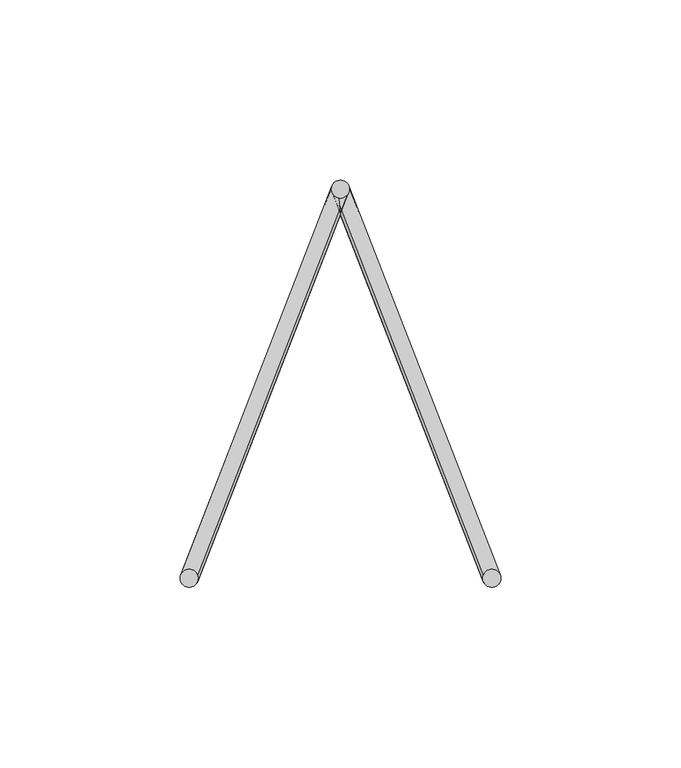
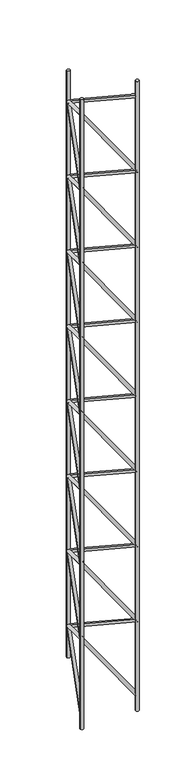
"""IFC4 building model written with IfcOpenShell, lengths in millimetres: proxy geometry, Pre-fab. (Vigota 4 - Pano 6)."""

import ifcopenshell
import ifcopenshell.guid

model = None  # the IFC model being written
_history = None  # IfcOwnerHistory: only IFC2X3 demands one
_inside = {}  # id of a spatial element -> (the spatial element, [elements in it])
_under = {}  # id of a project, library or spatial element -> (it, [spatial elements below it])
_declared = {}  # id of a project -> (the project, [libraries it declares])
_typed = {}  # id of a type object -> (the type object, [elements of that type])
_made_of = {}  # id of a material, layer set ... -> (it, [elements and type objects made of it])


def new_model(schema):
    """Start an empty IFC model of exactly this schema.

    Asked for "IFC4X3", IfcOpenShell would pick the latest addendum, in which some entities
    have other attributes; the version numbers below select the first issue.
    IFC2X3 requires an IfcOwnerHistory on every rooted entity: one is made here for all.
    """
    global model, _history
    if schema == "IFC4X3":
        model = ifcopenshell.file(schema_version=(4, 3, 0, 0))
    else:
        model = ifcopenshell.file(schema=schema)
    _inside.clear()
    _under.clear()
    _declared.clear()
    _typed.clear()
    _made_of.clear()
    _history = None
    if model.schema == "IFC2X3":
        org = make("IfcOrganization", Name="unknown")
        user = make(
            "IfcPersonAndOrganization",
            ThePerson=make("IfcPerson", FamilyName="unknown"),
            TheOrganization=org,
        )
        app = make(
            "IfcApplication",
            ApplicationDeveloper=org,
            Version="unknown",
            ApplicationFullName="unknown",
            ApplicationIdentifier="unknown",
        )
        _history = make(
            "IfcOwnerHistory",
            OwningUser=user,
            OwningApplication=app,
            ChangeAction="ADDED",
            CreationDate=0,
        )
    return model


def make(cls, **values):
    """One entity of the class cls with the attributes given. An attribute that is None is left unset."""
    return model.create_entity(
        cls, **{name: value for name, value in values.items() if value is not None}
    )


def rooted(cls, **values):
    """An entity with a GlobalId (a new one), such as an element, a storey or a relation."""
    return make(cls, GlobalId=ifcopenshell.guid.new(), OwnerHistory=_history, **values)


def si_unit(unit_type, name, prefix=None):
    """IfcSIUnit, for example si_unit("LENGTHUNIT", "METRE", prefix="MILLI")."""
    return make("IfcSIUnit", UnitType=unit_type, Prefix=prefix, Name=name)


def assignment(units):
    """IfcUnitAssignment: the units of a project."""
    return None if units is None else make("IfcUnitAssignment", Units=units)


def point(xyz):
    """IfcCartesianPoint."""
    return None if xyz is None else make("IfcCartesianPoint", Coordinates=xyz)


def direction(xyz):
    """IfcDirection."""
    return None if xyz is None else make("IfcDirection", DirectionRatios=xyz)


def frame(location, z_axis=None, x_axis=None):
    """IfcAxis2Placement3D, a coordinate frame: its origin and axes. An axis left out is left unset."""
    return make(
        "IfcAxis2Placement3D",
        Location=point(location),
        Axis=direction(z_axis),
        RefDirection=direction(x_axis),
    )


def frame_2d(location, x_axis=None):
    """IfcAxis2Placement2D, a coordinate frame in the plane: its origin and x axis."""
    return make(
        "IfcAxis2Placement2D", Location=point(location), RefDirection=direction(x_axis)
    )


def origin():
    """The frame at (0, 0, 0) with its axes left unset."""
    return frame((0.0, 0.0, 0.0))


def origin_with_axes():
    """The frame at (0, 0, 0) with the z axis (0, 0, 1) and the x axis (1, 0, 0) written out."""
    return frame((0.0, 0.0, 0.0), z_axis=(0.0, 0.0, 1.0), x_axis=(1.0, 0.0, 0.0))


def origin_2d():
    """The frame at (0, 0) in the plane with its x axis left unset."""
    return frame_2d((0.0, 0.0))


def place(relative_to, where):
    """IfcLocalPlacement: puts the frame where relative to a parent placement (None: the world)."""
    return make(
        "IfcLocalPlacement", PlacementRelTo=relative_to, RelativePlacement=where
    )


def context(
    kind, dimensions, precision=None, world=None, true_north=None, identifier=None
):
    """IfcGeometricRepresentationContext, for example the 3D "Model" context."""
    return make(
        "IfcGeometricRepresentationContext",
        ContextIdentifier=identifier,
        ContextType=kind,
        CoordinateSpaceDimension=dimensions,
        Precision=precision,
        WorldCoordinateSystem=world,
        TrueNorth=true_north,
    )


def project(units=None, contexts=None):
    """IfcProject with its units and contexts."""
    return rooted(
        "IfcProject",
        Name="project",
        RepresentationContexts=contexts,
        UnitsInContext=assignment(units),
    )


def spatial(cls, under=None, at=None, **own):
    """A site, building, storey or space (cls), placed at a placement, below another one or the project."""
    s = rooted(cls, ObjectPlacement=at, **own)
    if under is not None:
        _under.setdefault(under.id(), (under, []))[1].append(s)
    return s


def circle_curve(where, radius):
    """IfcCircle in the frame where."""
    return make("IfcCircle", Position=where, Radius=radius)


def trimmed(basis, trim1, trim2, sense, master):
    """IfcTrimmedCurve: the piece of a basis curve between two trims."""
    return make(
        "IfcTrimmedCurve",
        BasisCurve=basis,
        Trim1=trim1,
        Trim2=trim2,
        SenseAgreement=sense,
        MasterRepresentation=master,
    )


def segment(curve, same_sense, transition):
    """IfcCompositeCurveSegment."""
    return make(
        "IfcCompositeCurveSegment",
        Transition=transition,
        SameSense=same_sense,
        ParentCurve=curve,
    )


def composite_curve(segments, self_intersect=None):
    """IfcCompositeCurve: segments joined end to end."""
    return make("IfcCompositeCurve", Segments=segments, SelfIntersect=self_intersect)


def outline(outer, holes=None, kind="AREA"):
    """IfcArbitraryClosedProfileDef: a profile drawn as a closed curve; with holes, ...WithVoids."""
    if holes is None:
        return make("IfcArbitraryClosedProfileDef", ProfileType=kind, OuterCurve=outer)
    return make(
        "IfcArbitraryProfileDefWithVoids",
        ProfileType=kind,
        OuterCurve=outer,
        InnerCurves=holes,
    )


def extrude(swept, where, along, depth):
    """IfcExtrudedAreaSolid: the profile swept, set in the frame where, extruded along a direction by depth."""
    return make(
        "IfcExtrudedAreaSolid",
        SweptArea=swept,
        Position=where,
        ExtrudedDirection=direction(along),
        Depth=depth,
    )


def shape(context_of_items, identifier, shape_type, items):
    """IfcShapeRepresentation: the items that make up one representation, for example the "Body"."""
    return make(
        "IfcShapeRepresentation",
        ContextOfItems=context_of_items,
        RepresentationIdentifier=identifier,
        RepresentationType=shape_type,
        Items=items,
    )


def source(mapping_origin, context_of_items, identifier, shape_type, items):
    """IfcRepresentationMap: a shape defined once, which mapped items show again and again."""
    return make(
        "IfcRepresentationMap",
        MappingOrigin=mapping_origin,
        MappedRepresentation=shape(context_of_items, identifier, shape_type, items),
    )


def transform(
    local_origin,
    x_axis=None,
    y_axis=None,
    z_axis=None,
    scale=None,
    scale2=None,
    scale3=None,
    uniform=True,
):
    """IfcCartesianTransformationOperator3D, or its non-uniform kind. x_axis, y_axis, z_axis: its Axis1, 2, 3."""
    if uniform:
        return make(
            "IfcCartesianTransformationOperator3D",
            Axis1=direction(x_axis),
            Axis2=direction(y_axis),
            LocalOrigin=point(local_origin),
            Scale=scale,
            Axis3=direction(z_axis),
        )
    return make(
        "IfcCartesianTransformationOperator3DnonUniform",
        Axis1=direction(x_axis),
        Axis2=direction(y_axis),
        LocalOrigin=point(local_origin),
        Scale=scale,
        Axis3=direction(z_axis),
        Scale2=scale2,
        Scale3=scale3,
    )


def mapped(mapping_source, mapping_target):
    """IfcMappedItem: shows the shape of a source again, moved by a transform."""
    return make(
        "IfcMappedItem", MappingSource=mapping_source, MappingTarget=mapping_target
    )


def made_of(thing, what):
    """Note that an element or type object is made of a material, layer set ...; save() writes the relation."""
    if what is not None:
        _made_of.setdefault(what.id(), (what, []))[1].append(thing)
    return thing


def element(
    cls,
    number,
    at=None,
    inside=None,
    cuts=None,
    type_object=None,
    material=None,
    context=None,
    identifier="Body",
    shape_type=None,
    held_by="IfcProductDefinitionShape",
    body=None,
    shapes=None,
    **own,
):
    """One element of the class cls, such as IfcWall. Its Tag is "e" and its number.

    at: its placement. inside: the storey or other place that contains it. cuts: it is an
    opening in that element (IfcRelVoidsElement). A single representation is given by context,
    identifier, shape_type and body (its items); several are given by shapes. held_by: the class
    of the entity that holds the representations. save() writes the other relations.
    """
    e = rooted(cls, Tag="e%d" % number, ObjectPlacement=at, **own)
    if body is not None:
        shapes = [shape(context, identifier, shape_type, body)]
    if shapes is not None:
        e.Representation = make(held_by, Representations=shapes)
    if inside is not None:
        _inside.setdefault(inside.id(), (inside, []))[1].append(e)
    if cuts is not None:
        rooted(
            "IfcRelVoidsElement", RelatingBuildingElement=cuts, RelatedOpeningElement=e
        )
    if type_object is not None:
        _typed.setdefault(type_object.id(), (type_object, []))[1].append(e)
    return made_of(e, material)


def aggregate(whole, parts):
    """IfcRelAggregates: a whole, such as a stair, and the parts it consists of."""
    return rooted("IfcRelAggregates", RelatingObject=whole, RelatedObjects=parts)


def save(model, path):
    """Write the relations noted so far, then the file.

    IfcRelAggregates (storeys below a building ...), IfcRelContainedInSpatialStructure (elements
    in a storey), IfcRelDefinesByType, IfcRelAssociatesMaterial and IfcRelDeclares: one each for
    every whole, place, type object, material and project.
    """
    for whole, parts in _under.values():
        aggregate(whole, parts)
    for where, things in _inside.values():
        rooted(
            "IfcRelContainedInSpatialStructure",
            RelatedElements=things,
            RelatingStructure=where,
        )
    for kind, things in _typed.values():
        rooted("IfcRelDefinesByType", RelatedObjects=things, RelatingType=kind)
    for what, things in _made_of.values():
        rooted("IfcRelAssociatesMaterial", RelatedObjects=things, RelatingMaterial=what)
    for by, libraries in _declared.values():
        rooted("IfcRelDeclares", RelatingContext=by, RelatedDefinitions=libraries)
    model.write(path)


def structural_framing_ea5c50d0(model_context):
    return source(origin(), model_context, "Body", "SweptSolid", [
        extrude(outline(composite_curve([segment(trimmed(circle_curve(origin_2d(), 2.5), [point((2.5, 0.0))], [point((-2.5, 0.0))], False, "CARTESIAN"), True, "CONTINUOUS"), segment(trimmed(circle_curve(origin_2d(), 2.5), [point((-2.5, 0.0))], [point((2.5, 0.0))], False, "CARTESIAN"), True, "CONTINUOUS")], self_intersect=False)), origin_with_axes(), (0.0, 0.0, 1.0), 1009.0),
        extrude(outline(composite_curve([segment(trimmed(circle_curve(frame_2d((-42.0, 108.0)), 2.5), [point((-39.5, 108.0))], [point((-44.5, 108.0))], False, "CARTESIAN"), True, "CONTINUOUS"), segment(trimmed(circle_curve(frame_2d((-42.0, 108.0)), 2.5), [point((-44.5, 108.0))], [point((-39.5, 108.0))], False, "CARTESIAN"), True, "CONTINUOUS")], self_intersect=False)), frame((0.0, 0.0, 34.5), z_axis=(0.0, 0.0, 1.0), x_axis=(1.0, 0.0, 0.0)), (0.0, 0.0, 1.0), 940.0),
        extrude(outline(composite_curve([segment(trimmed(circle_curve(origin_2d(), 2.5), [point((2.5, 0.0))], [point((-2.5, 0.0))], False, "CARTESIAN"), True, "CONTINUOUS"), segment(trimmed(circle_curve(origin_2d(), 2.5), [point((-2.5, 0.0))], [point((2.5, 0.0))], False, "CARTESIAN"), True, "CONTINUOUS")], self_intersect=False)), frame((0.0, 0.0, 24.5), z_axis=(-0.3218603428886276, 0.8276408817707567, 0.4598004898837537), x_axis=(0.8192319205108605, -3.936835275445103e-11, 0.5734623443750141)), (0.0, 0.0, 1.0), 130.491379),
        extrude(outline(composite_curve([segment(trimmed(circle_curve(origin_2d(), 2.5), [point((2.5, 0.0))], [point((-2.5, 0.0))], False, "CARTESIAN"), True, "CONTINUOUS"), segment(trimmed(circle_curve(origin_2d(), 2.5), [point((-2.5, 0.0))], [point((2.5, 0.0))], False, "CARTESIAN"), True, "CONTINUOUS")], self_intersect=False)), frame((-42.0, 108.0, 84.5), z_axis=(0.3218603428886276, -0.8276408817707567, 0.4598004898837537), x_axis=(0.8192319205108605, -3.936835275445103e-11, -0.5734623443750141)), (0.0, 0.0, 1.0), 130.491379),
        extrude(outline(composite_curve([segment(trimmed(circle_curve(origin_2d(), 2.5), [point((2.5, 0.0))], [point((-2.5, 0.0))], False, "CARTESIAN"), True, "CONTINUOUS"), segment(trimmed(circle_curve(origin_2d(), 2.5), [point((-2.5, 0.0))], [point((2.5, 0.0))], False, "CARTESIAN"), True, "CONTINUOUS")], self_intersect=False)), frame((0.0, 0.0, 144.5), z_axis=(-0.3218603428886276, 0.8276408817707567, 0.4598004898837537), x_axis=(0.8192319205108605, -3.936835275445103e-11, 0.5734623443750141)), (0.0, 0.0, 1.0), 130.491379),
        extrude(outline(composite_curve([segment(trimmed(circle_curve(origin_2d(), 2.5), [point((2.5, 0.0))], [point((-2.5, 0.0))], False, "CARTESIAN"), True, "CONTINUOUS"), segment(trimmed(circle_curve(origin_2d(), 2.5), [point((-2.5, 0.0))], [point((2.5, 0.0))], False, "CARTESIAN"), True, "CONTINUOUS")], self_intersect=False)), frame((-42.0, 108.0, 204.5), z_axis=(0.3218603428886276, -0.8276408817707567, 0.4598004898837537), x_axis=(0.8192319205108605, -3.936835275445103e-11, -0.5734623443750141)), (0.0, 0.0, 1.0), 130.491379),
        extrude(outline(composite_curve([segment(trimmed(circle_curve(origin_2d(), 2.5), [point((2.5, 0.0))], [point((-2.5, 0.0))], False, "CARTESIAN"), True, "CONTINUOUS"), segment(trimmed(circle_curve(origin_2d(), 2.5), [point((-2.5, 0.0))], [point((2.5, 0.0))], False, "CARTESIAN"), True, "CONTINUOUS")], self_intersect=False)), frame((0.0, 0.0, 264.5), z_axis=(-0.3218603428886276, 0.8276408817707567, 0.4598004898837537), x_axis=(0.8192319205108605, -3.936835275445103e-11, 0.5734623443750141)), (0.0, 0.0, 1.0), 130.491379),
        extrude(outline(composite_curve([segment(trimmed(circle_curve(origin_2d(), 2.5), [point((2.5, 0.0))], [point((-2.5, 0.0))], False, "CARTESIAN"), True, "CONTINUOUS"), segment(trimmed(circle_curve(origin_2d(), 2.5), [point((-2.5, 0.0))], [point((2.5, 0.0))], False, "CARTESIAN"), True, "CONTINUOUS")], self_intersect=False)), frame((-42.0, 108.0, 324.5), z_axis=(0.3218603428886276, -0.8276408817707567, 0.4598004898837537), x_axis=(0.8192319205108605, -3.936835275445103e-11, -0.5734623443750141)), (0.0, 0.0, 1.0), 130.491379),
        extrude(outline(composite_curve([segment(trimmed(circle_curve(origin_2d(), 2.5), [point((2.5, 0.0))], [point((-2.5, 0.0))], False, "CARTESIAN"), True, "CONTINUOUS"), segment(trimmed(circle_curve(origin_2d(), 2.5), [point((-2.5, 0.0))], [point((2.5, 0.0))], False, "CARTESIAN"), True, "CONTINUOUS")], self_intersect=False)), frame((0.0, 0.0, 384.5), z_axis=(-0.3218603428886276, 0.8276408817707567, 0.4598004898837537), x_axis=(0.8192319205108605, -3.936835275445103e-11, 0.5734623443750141)), (0.0, 0.0, 1.0), 130.491379),
        extrude(outline(composite_curve([segment(trimmed(circle_curve(origin_2d(), 2.5), [point((2.5, 0.0))], [point((-2.5, 0.0))], False, "CARTESIAN"), True, "CONTINUOUS"), segment(trimmed(circle_curve(origin_2d(), 2.5), [point((-2.5, 0.0))], [point((2.5, 0.0))], False, "CARTESIAN"), True, "CONTINUOUS")], self_intersect=False)), frame((-42.0, 108.0, 444.5), z_axis=(0.3218603428886276, -0.8276408817707567, 0.4598004898837537), x_axis=(0.8192319205108605, -3.936835275445103e-11, -0.5734623443750141)), (0.0, 0.0, 1.0), 130.491379),
        extrude(outline(composite_curve([segment(trimmed(circle_curve(origin_2d(), 2.5), [point((2.5, 0.0))], [point((-2.5, 0.0))], False, "CARTESIAN"), True, "CONTINUOUS"), segment(trimmed(circle_curve(origin_2d(), 2.5), [point((-2.5, 0.0))], [point((2.5, 0.0))], False, "CARTESIAN"), True, "CONTINUOUS")], self_intersect=False)), frame((0.0, 0.0, 504.5), z_axis=(-0.3218603428886276, 0.8276408817707567, 0.4598004898837537), x_axis=(0.8192319205108605, -3.936835275445103e-11, 0.5734623443750141)), (0.0, 0.0, 1.0), 130.491379),
        extrude(outline(composite_curve([segment(trimmed(circle_curve(origin_2d(), 2.5), [point((2.5, 0.0))], [point((-2.5, 0.0))], False, "CARTESIAN"), True, "CONTINUOUS"), segment(trimmed(circle_curve(origin_2d(), 2.5), [point((-2.5, 0.0))], [point((2.5, 0.0))], False, "CARTESIAN"), True, "CONTINUOUS")], self_intersect=False)), frame((-42.0, 108.0, 564.5), z_axis=(0.3218603428886276, -0.8276408817707567, 0.4598004898837537), x_axis=(0.8192319205108605, -3.936835275445103e-11, -0.5734623443750141)), (0.0, 0.0, 1.0), 130.491379),
        extrude(outline(composite_curve([segment(trimmed(circle_curve(origin_2d(), 2.5), [point((2.5, 0.0))], [point((-2.5, 0.0))], False, "CARTESIAN"), True, "CONTINUOUS"), segment(trimmed(circle_curve(origin_2d(), 2.5), [point((-2.5, 0.0))], [point((2.5, 0.0))], False, "CARTESIAN"), True, "CONTINUOUS")], self_intersect=False)), frame((0.0, 0.0, 624.5), z_axis=(-0.3218603428886276, 0.8276408817707567, 0.4598004898837537), x_axis=(0.8192319205108605, -3.936835275445103e-11, 0.5734623443750141)), (0.0, 0.0, 1.0), 130.491379),
        extrude(outline(composite_curve([segment(trimmed(circle_curve(origin_2d(), 2.5), [point((2.5, 0.0))], [point((-2.5, 0.0))], False, "CARTESIAN"), True, "CONTINUOUS"), segment(trimmed(circle_curve(origin_2d(), 2.5), [point((-2.5, 0.0))], [point((2.5, 0.0))], False, "CARTESIAN"), True, "CONTINUOUS")], self_intersect=False)), frame((-42.0, 108.0, 684.5), z_axis=(0.3218603428886276, -0.8276408817707567, 0.4598004898837537), x_axis=(0.8192319205108605, -3.936835275445103e-11, -0.5734623443750141)), (0.0, 0.0, 1.0), 130.491379),
        extrude(outline(composite_curve([segment(trimmed(circle_curve(origin_2d(), 2.5), [point((2.5, 0.0))], [point((-2.5, 0.0))], False, "CARTESIAN"), True, "CONTINUOUS"), segment(trimmed(circle_curve(origin_2d(), 2.5), [point((-2.5, 0.0))], [point((2.5, 0.0))], False, "CARTESIAN"), True, "CONTINUOUS")], self_intersect=False)), frame((0.0, 0.0, 744.5), z_axis=(-0.3218603428886276, 0.8276408817707567, 0.4598004898837537), x_axis=(0.8192319205108605, -3.936835275445103e-11, 0.5734623443750141)), (0.0, 0.0, 1.0), 130.491379),
        extrude(outline(composite_curve([segment(trimmed(circle_curve(origin_2d(), 2.5), [point((2.5, 0.0))], [point((-2.5, 0.0))], False, "CARTESIAN"), True, "CONTINUOUS"), segment(trimmed(circle_curve(origin_2d(), 2.5), [point((-2.5, 0.0))], [point((2.5, 0.0))], False, "CARTESIAN"), True, "CONTINUOUS")], self_intersect=False)), frame((-42.0, 108.0, 804.5), z_axis=(0.3218603428886276, -0.8276408817707567, 0.4598004898837537), x_axis=(0.8192319205108605, -3.936835275445103e-11, -0.5734623443750141)), (0.0, 0.0, 1.0), 130.491379),
        extrude(outline(composite_curve([segment(trimmed(circle_curve(origin_2d(), 2.5), [point((2.5, 0.0))], [point((-2.5, 0.0))], False, "CARTESIAN"), True, "CONTINUOUS"), segment(trimmed(circle_curve(origin_2d(), 2.5), [point((-2.5, 0.0))], [point((2.5, 0.0))], False, "CARTESIAN"), True, "CONTINUOUS")], self_intersect=False)), frame((0.0, 0.0, 864.5), z_axis=(-0.3218603428886276, 0.8276408817707567, 0.4598004898837537), x_axis=(0.8192319205108605, -3.936835275445103e-11, 0.5734623443750141)), (0.0, 0.0, 1.0), 130.491379),
        extrude(outline(composite_curve([segment(trimmed(circle_curve(origin_2d(), 2.5), [point((2.5, 0.0))], [point((-2.5, 0.0))], False, "CARTESIAN"), True, "CONTINUOUS"), segment(trimmed(circle_curve(origin_2d(), 2.5), [point((-2.5, 0.0))], [point((2.5, 0.0))], False, "CARTESIAN"), True, "CONTINUOUS")], self_intersect=False)), frame((-42.0, 108.0, 924.5), z_axis=(0.3218603428886276, -0.8276408817707567, 0.4598004898837537), x_axis=(0.8192319205108605, -3.936835275445103e-11, -0.5734623443750141)), (0.0, 0.0, 1.0), 130.491379),
        extrude(outline(composite_curve([segment(trimmed(circle_curve(frame_2d((-84.0, 0.0)), 2.5), [point((-81.5, 0.0))], [point((-86.5, 0.0))], False, "CARTESIAN"), True, "CONTINUOUS"), segment(trimmed(circle_curve(frame_2d((-84.0, 0.0)), 2.5), [point((-86.5, 0.0))], [point((-81.5, 0.0))], False, "CARTESIAN"), True, "CONTINUOUS")], self_intersect=False)), origin_with_axes(), (0.0, 0.0, 1.0), 1009.0),
        extrude(outline(composite_curve([segment(trimmed(circle_curve(origin_2d(), 2.5), [point((2.5, 0.0))], [point((-2.5, 0.0))], False, "CARTESIAN"), True, "CONTINUOUS"), segment(trimmed(circle_curve(origin_2d(), 2.5), [point((-2.5, 0.0))], [point((2.5, 0.0))], False, "CARTESIAN"), True, "CONTINUOUS")], self_intersect=False)), frame((-84.0, 0.0, 24.5), z_axis=(0.3218603428886276, 0.8276408817707567, 0.4598004898837537), x_axis=(0.8192319205108605, 3.936835275445103e-11, -0.5734623443750141)), (0.0, 0.0, 1.0), 130.491379),
        extrude(outline(composite_curve([segment(trimmed(circle_curve(origin_2d(), 2.5), [point((2.5, 0.0))], [point((-2.5, 0.0))], False, "CARTESIAN"), True, "CONTINUOUS"), segment(trimmed(circle_curve(origin_2d(), 2.5), [point((-2.5, 0.0))], [point((2.5, 0.0))], False, "CARTESIAN"), True, "CONTINUOUS")], self_intersect=False)), frame((-42.0, 108.0, 84.5), z_axis=(-0.3218603428886276, -0.8276408817707567, 0.4598004898837537), x_axis=(0.8192319205108605, 3.936835275445103e-11, 0.5734623443750141)), (0.0, 0.0, 1.0), 130.491379),
        extrude(outline(composite_curve([segment(trimmed(circle_curve(origin_2d(), 2.5), [point((2.5, 0.0))], [point((-2.5, 0.0))], False, "CARTESIAN"), True, "CONTINUOUS"), segment(trimmed(circle_curve(origin_2d(), 2.5), [point((-2.5, 0.0))], [point((2.5, 0.0))], False, "CARTESIAN"), True, "CONTINUOUS")], self_intersect=False)), frame((-84.0, 0.0, 144.5), z_axis=(0.3218603428886276, 0.8276408817707567, 0.4598004898837537), x_axis=(0.8192319205108605, 3.936835275445103e-11, -0.5734623443750141)), (0.0, 0.0, 1.0), 130.491379),
        extrude(outline(composite_curve([segment(trimmed(circle_curve(origin_2d(), 2.5), [point((2.5, 0.0))], [point((-2.5, 0.0))], False, "CARTESIAN"), True, "CONTINUOUS"), segment(trimmed(circle_curve(origin_2d(), 2.5), [point((-2.5, 0.0))], [point((2.5, 0.0))], False, "CARTESIAN"), True, "CONTINUOUS")], self_intersect=False)), frame((-42.0, 108.0, 204.5), z_axis=(-0.3218603428886276, -0.8276408817707567, 0.4598004898837537), x_axis=(0.8192319205108605, 3.936835275445103e-11, 0.5734623443750141)), (0.0, 0.0, 1.0), 130.491379),
        extrude(outline(composite_curve([segment(trimmed(circle_curve(origin_2d(), 2.5), [point((2.5, 0.0))], [point((-2.5, 0.0))], False, "CARTESIAN"), True, "CONTINUOUS"), segment(trimmed(circle_curve(origin_2d(), 2.5), [point((-2.5, 0.0))], [point((2.5, 0.0))], False, "CARTESIAN"), True, "CONTINUOUS")], self_intersect=False)), frame((-84.0, 0.0, 264.5), z_axis=(0.3218603428886276, 0.8276408817707567, 0.4598004898837537), x_axis=(0.8192319205108605, 3.936835275445103e-11, -0.5734623443750141)), (0.0, 0.0, 1.0), 130.491379),
        extrude(outline(composite_curve([segment(trimmed(circle_curve(origin_2d(), 2.5), [point((2.5, 0.0))], [point((-2.5, 0.0))], False, "CARTESIAN"), True, "CONTINUOUS"), segment(trimmed(circle_curve(origin_2d(), 2.5), [point((-2.5, 0.0))], [point((2.5, 0.0))], False, "CARTESIAN"), True, "CONTINUOUS")], self_intersect=False)), frame((-42.0, 108.0, 324.5), z_axis=(-0.3218603428886276, -0.8276408817707567, 0.4598004898837537), x_axis=(0.8192319205108605, 3.936835275445103e-11, 0.5734623443750141)), (0.0, 0.0, 1.0), 130.491379),
        extrude(outline(composite_curve([segment(trimmed(circle_curve(origin_2d(), 2.5), [point((2.5, 0.0))], [point((-2.5, 0.0))], False, "CARTESIAN"), True, "CONTINUOUS"), segment(trimmed(circle_curve(origin_2d(), 2.5), [point((-2.5, 0.0))], [point((2.5, 0.0))], False, "CARTESIAN"), True, "CONTINUOUS")], self_intersect=False)), frame((-84.0, 0.0, 384.5), z_axis=(0.3218603428886276, 0.8276408817707567, 0.4598004898837537), x_axis=(0.8192319205108605, 3.936835275445103e-11, -0.5734623443750141)), (0.0, 0.0, 1.0), 130.491379),
        extrude(outline(composite_curve([segment(trimmed(circle_curve(origin_2d(), 2.5), [point((2.5, 0.0))], [point((-2.5, 0.0))], False, "CARTESIAN"), True, "CONTINUOUS"), segment(trimmed(circle_curve(origin_2d(), 2.5), [point((-2.5, 0.0))], [point((2.5, 0.0))], False, "CARTESIAN"), True, "CONTINUOUS")], self_intersect=False)), frame((-42.0, 108.0, 444.5), z_axis=(-0.3218603428886276, -0.8276408817707567, 0.4598004898837537), x_axis=(0.8192319205108605, 3.936835275445103e-11, 0.5734623443750141)), (0.0, 0.0, 1.0), 130.491379),
        extrude(outline(composite_curve([segment(trimmed(circle_curve(origin_2d(), 2.5), [point((2.5, 0.0))], [point((-2.5, 0.0))], False, "CARTESIAN"), True, "CONTINUOUS"), segment(trimmed(circle_curve(origin_2d(), 2.5), [point((-2.5, 0.0))], [point((2.5, 0.0))], False, "CARTESIAN"), True, "CONTINUOUS")], self_intersect=False)), frame((-84.0, 0.0, 504.5), z_axis=(0.3218603428886276, 0.8276408817707567, 0.4598004898837537), x_axis=(0.8192319205108605, 3.936835275445103e-11, -0.5734623443750141)), (0.0, 0.0, 1.0), 130.491379),
        extrude(outline(composite_curve([segment(trimmed(circle_curve(origin_2d(), 2.5), [point((2.5, 0.0))], [point((-2.5, 0.0))], False, "CARTESIAN"), True, "CONTINUOUS"), segment(trimmed(circle_curve(origin_2d(), 2.5), [point((-2.5, 0.0))], [point((2.5, 0.0))], False, "CARTESIAN"), True, "CONTINUOUS")], self_intersect=False)), frame((-42.0, 108.0, 564.5), z_axis=(-0.3218603428886276, -0.8276408817707567, 0.4598004898837537), x_axis=(0.8192319205108605, 3.936835275445103e-11, 0.5734623443750141)), (0.0, 0.0, 1.0), 130.491379),
        extrude(outline(composite_curve([segment(trimmed(circle_curve(origin_2d(), 2.5), [point((2.5, 0.0))], [point((-2.5, 0.0))], False, "CARTESIAN"), True, "CONTINUOUS"), segment(trimmed(circle_curve(origin_2d(), 2.5), [point((-2.5, 0.0))], [point((2.5, 0.0))], False, "CARTESIAN"), True, "CONTINUOUS")], self_intersect=False)), frame((-84.0, 0.0, 624.5), z_axis=(0.3218603428886276, 0.8276408817707567, 0.4598004898837537), x_axis=(0.8192319205108605, 3.936835275445103e-11, -0.5734623443750141)), (0.0, 0.0, 1.0), 130.491379),
        extrude(outline(composite_curve([segment(trimmed(circle_curve(origin_2d(), 2.5), [point((2.5, 0.0))], [point((-2.5, 0.0))], False, "CARTESIAN"), True, "CONTINUOUS"), segment(trimmed(circle_curve(origin_2d(), 2.5), [point((-2.5, 0.0))], [point((2.5, 0.0))], False, "CARTESIAN"), True, "CONTINUOUS")], self_intersect=False)), frame((-42.0, 108.0, 684.5), z_axis=(-0.3218603428886276, -0.8276408817707567, 0.4598004898837537), x_axis=(0.8192319205108605, 3.936835275445103e-11, 0.5734623443750141)), (0.0, 0.0, 1.0), 130.491379),
        extrude(outline(composite_curve([segment(trimmed(circle_curve(origin_2d(), 2.5), [point((2.5, 0.0))], [point((-2.5, 0.0))], False, "CARTESIAN"), True, "CONTINUOUS"), segment(trimmed(circle_curve(origin_2d(), 2.5), [point((-2.5, 0.0))], [point((2.5, 0.0))], False, "CARTESIAN"), True, "CONTINUOUS")], self_intersect=False)), frame((-84.0, 0.0, 744.5), z_axis=(0.3218603428886276, 0.8276408817707567, 0.4598004898837537), x_axis=(0.8192319205108605, 3.936835275445103e-11, -0.5734623443750141)), (0.0, 0.0, 1.0), 130.491379),
        extrude(outline(composite_curve([segment(trimmed(circle_curve(origin_2d(), 2.5), [point((2.5, 0.0))], [point((-2.5, 0.0))], False, "CARTESIAN"), True, "CONTINUOUS"), segment(trimmed(circle_curve(origin_2d(), 2.5), [point((-2.5, 0.0))], [point((2.5, 0.0))], False, "CARTESIAN"), True, "CONTINUOUS")], self_intersect=False)), frame((-42.0, 108.0, 804.5), z_axis=(-0.3218603428886276, -0.8276408817707567, 0.4598004898837537), x_axis=(0.8192319205108605, 3.936835275445103e-11, 0.5734623443750141)), (0.0, 0.0, 1.0), 130.491379),
        extrude(outline(composite_curve([segment(trimmed(circle_curve(origin_2d(), 2.5), [point((2.5, 0.0))], [point((-2.5, 0.0))], False, "CARTESIAN"), True, "CONTINUOUS"), segment(trimmed(circle_curve(origin_2d(), 2.5), [point((-2.5, 0.0))], [point((2.5, 0.0))], False, "CARTESIAN"), True, "CONTINUOUS")], self_intersect=False)), frame((-84.0, 0.0, 864.5), z_axis=(0.3218603428886276, 0.8276408817707567, 0.4598004898837537), x_axis=(0.8192319205108605, 3.936835275445103e-11, -0.5734623443750141)), (0.0, 0.0, 1.0), 130.491379),
        extrude(outline(composite_curve([segment(trimmed(circle_curve(origin_2d(), 2.5), [point((2.5, 0.0))], [point((-2.5, 0.0))], False, "CARTESIAN"), True, "CONTINUOUS"), segment(trimmed(circle_curve(origin_2d(), 2.5), [point((-2.5, 0.0))], [point((2.5, 0.0))], False, "CARTESIAN"), True, "CONTINUOUS")], self_intersect=False)), frame((-42.0, 108.0, 924.5), z_axis=(-0.3218603428886276, -0.8276408817707567, 0.4598004898837537), x_axis=(0.8192319205108605, 3.936835275445103e-11, 0.5734623443750141)), (0.0, 0.0, 1.0), 130.491379),
    ])


if __name__ == "__main__":
    model = new_model("IFC4")
    model_context = context("Model", 3, world=origin())
    ifc_project = project(units=[si_unit("LENGTHUNIT", "METRE", prefix="MILLI")], contexts=[model_context])
    site = spatial("IfcSite", under=ifc_project)
    building = spatial("IfcBuilding", under=site)
    placement = place(None, origin())
    structural_framing_shape = structural_framing_ea5c50d0(model_context)
    element("IfcBuildingElementProxy", 1, Name="Pre-fab. (Vigota 4 - Pano 6)", ObjectType="Pre-fab. (Vigota 4 - Pano 6)", at=placement, inside=building, context=model_context, shape_type="MappedRepresentation", body=[
        mapped(structural_framing_shape, transform((0.0, 0.0, 0.0), x_axis=(1.0, 0.0, 0.0), y_axis=(0.0, 1.0, 0.0), z_axis=(0.0, 0.0, 1.0))),
    ])
    save(model, "model.ifc")

# Revit data of these elements
# Element 1 (IfcBuildingElementProxy, "Pre-fab. (Vigota 4 - Pano 6)")
#   Materials on its faces: "Aço"
# Materials
#   "Aço": class "Metal", colour RGB 120 120 120, transparency 0, Description = "Aço estrutural A36 grau, ASTM B, acabamento laminado", Cost = 0
